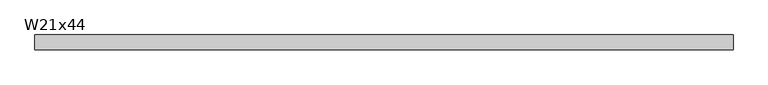
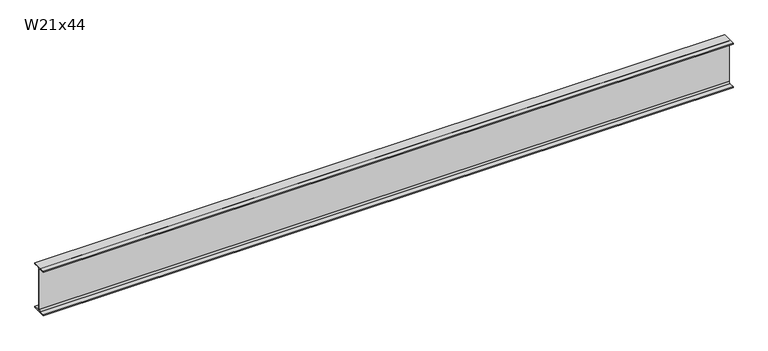
"""IFC4 building model written with IfcOpenShell, lengths in millimetres: beam geometry, RME W-Wide Flange : W21x44."""

from ifc_helpers import new_model, si_unit, point, frame, frame_2d, origin, place, context, project, spatial, polyline, circle_curve, trimmed, segment, composite_curve, outline, extrude, source, transform, mapped, element, save


def w21x44_f86bf4de(model_context):
    return source(origin(), model_context, "Body", "SweptSolid", [
        extrude(outline(composite_curve([segment(polyline([(82.55, -251.46), (82.55, -262.89), (-82.55, -262.89), (-82.55, -251.46), (-21.59, -251.46)]), True, "CONTINUOUS"), segment(trimmed(circle_curve(frame_2d((-21.59, -234.315)), 17.145), [point((-21.59, -251.46))], [point((-4.445, -234.315))], True, "CARTESIAN"), True, "CONTINUOUS"), segment(polyline([(-4.445, -234.315), (-4.445, 234.315)]), True, "CONTINUOUS"), segment(trimmed(circle_curve(frame_2d((-21.59, 234.315)), 17.145), [point((-4.445, 234.315))], [point((-21.59, 251.46))], True, "CARTESIAN"), True, "CONTINUOUS"), segment(polyline([(-21.59, 251.46), (-82.55, 251.46), (-82.55, 262.89), (82.55, 262.89), (82.55, 251.46), (21.59, 251.46)]), True, "CONTINUOUS"), segment(trimmed(circle_curve(frame_2d((21.59, 234.315)), 17.145), [point((21.59, 251.46))], [point((4.445, 234.315))], True, "CARTESIAN"), True, "CONTINUOUS"), segment(polyline([(4.445, 234.315), (4.445, -234.315)]), True, "CONTINUOUS"), segment(trimmed(circle_curve(frame_2d((21.59, -234.315)), 17.145), [point((4.445, -234.315))], [point((21.59, -251.46))], True, "CARTESIAN"), True, "CONTINUOUS"), segment(polyline([(21.59, -251.46), (82.55, -251.46)]), True, "CONTINUOUS")], self_intersect=False)), frame((-3876.6154311, 0.0, 0.0), z_axis=(1.0, 0.0, 0.0), x_axis=(0.0, 1.0, 0.0)), (0.0, 0.0, 1.0), 7709.535),
    ])


if __name__ == "__main__":
    model = new_model("IFC4")
    model_context = context("Model", 3, world=origin())
    ifc_project = project(units=[si_unit("LENGTHUNIT", "METRE", prefix="MILLI")], contexts=[model_context])
    site = spatial("IfcSite", under=ifc_project)
    building = spatial("IfcBuilding", under=site)
    placement = place(None, origin())
    w21x44_shape = w21x44_f86bf4de(model_context)
    element("IfcBeam", 1, ObjectType="RME W-Wide Flange : W21x44", at=placement, inside=building, context=model_context, shape_type="MappedRepresentation", body=[
        mapped(w21x44_shape, transform((0.0, 0.0, 0.0), x_axis=(1.0, 0.0, 0.0), y_axis=(0.0, 1.0, 0.0), z_axis=(0.0, 0.0, 1.0))),
    ])
    save(model, "model.ifc")

# Revit data of these elements
# Type "RME W-Wide Flange : W21x44"
#   WELD P [instance default] = ""
#   WELD LE [instance default] = ""
#   WELD D [instance default] = ""
#   TOP SECTION SIZE [instance default] = ""
#   TOP SECTION LENGTH [instance default] = ""
#   REMARKS [instance default] = ""
#   REINF TYPE [instance default] = ""
#   Nominal Size = "W24"
#   End Bearing Capacity [instance default] = ""
#   BOT SECTION SIZE [instance default] = ""
#   BOT SECTION LENGTH [instance default] = ""
#   Assembly Code = "B10"
#   W = 44
#   Start Extension Calculation [instance default] = 10' - 0"
#   Start Extension [instance default] = -0' - 0 1/2"
#   End Extension Calculation [instance default] = 10' - 0"
#   End Extension [instance default] = -0' - 0 1/2"
#   Length [instance default] = 5' - 0"
#   bf = 0' - 6 1/2"
#   d = 1' - 8.7"
#   k = 0' - 1 1/8"
#   k2 = 0' - 0.675"
#   tf = 0' - 0.45"
#   tw = 0' - 0.35"
#   A = 0.0902778 SF
#   Structural Material [instance default] = Metal - Steel - ASTM A992
# Element 1 (IfcBeam, "RME W-Wide Flange : W21x44")
#   Length = 26' - 1.00469"
#   Materials on its faces: "Metal - Steel - ASTM A992"
# Materials
#   "Metal - Steel - ASTM A992": class "Metal", colour RGB 255 128 0, transparency 0
